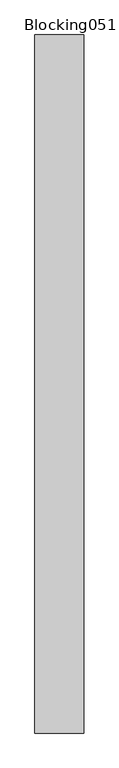
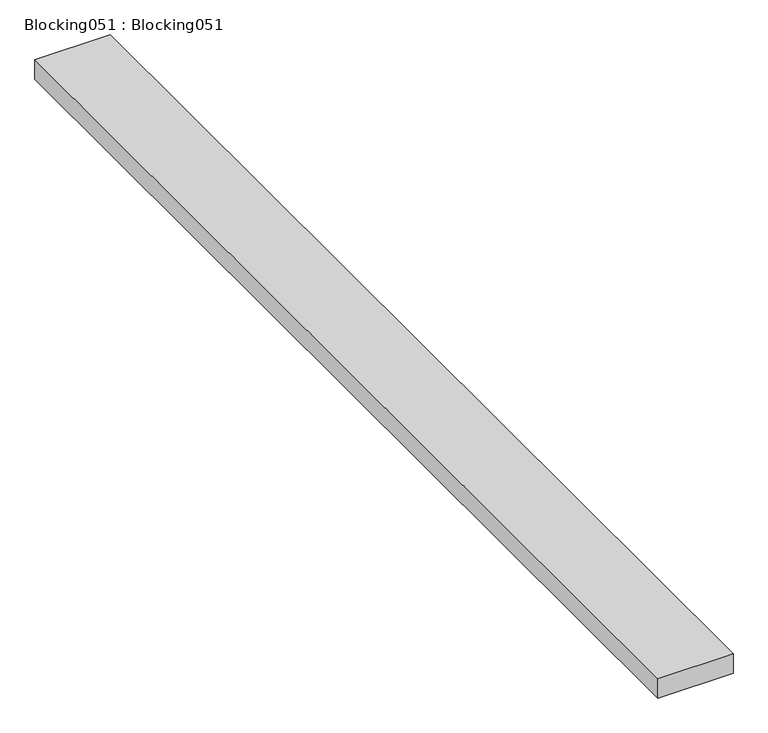
"""IFC4 building model written with IfcOpenShell, lengths in millimetres: proxy geometry, Blocking051 : Blocking051."""

import ifcopenshell
import ifcopenshell.guid

model = None  # the IFC model being written
_history = None  # IfcOwnerHistory: only IFC2X3 demands one
_inside = {}  # id of a spatial element -> (the spatial element, [elements in it])
_under = {}  # id of a project, library or spatial element -> (it, [spatial elements below it])
_declared = {}  # id of a project -> (the project, [libraries it declares])
_typed = {}  # id of a type object -> (the type object, [elements of that type])
_made_of = {}  # id of a material, layer set ... -> (it, [elements and type objects made of it])


def new_model(schema):
    """Start an empty IFC model of exactly this schema.

    Asked for "IFC4X3", IfcOpenShell would pick the latest addendum, in which some entities
    have other attributes; the version numbers below select the first issue.
    IFC2X3 requires an IfcOwnerHistory on every rooted entity: one is made here for all.
    """
    global model, _history
    if schema == "IFC4X3":
        model = ifcopenshell.file(schema_version=(4, 3, 0, 0))
    else:
        model = ifcopenshell.file(schema=schema)
    _inside.clear()
    _under.clear()
    _declared.clear()
    _typed.clear()
    _made_of.clear()
    _history = None
    if model.schema == "IFC2X3":
        org = make("IfcOrganization", Name="unknown")
        user = make(
            "IfcPersonAndOrganization",
            ThePerson=make("IfcPerson", FamilyName="unknown"),
            TheOrganization=org,
        )
        app = make(
            "IfcApplication",
            ApplicationDeveloper=org,
            Version="unknown",
            ApplicationFullName="unknown",
            ApplicationIdentifier="unknown",
        )
        _history = make(
            "IfcOwnerHistory",
            OwningUser=user,
            OwningApplication=app,
            ChangeAction="ADDED",
            CreationDate=0,
        )
    return model


def make(cls, **values):
    """One entity of the class cls with the attributes given. An attribute that is None is left unset."""
    return model.create_entity(
        cls, **{name: value for name, value in values.items() if value is not None}
    )


def rooted(cls, **values):
    """An entity with a GlobalId (a new one), such as an element, a storey or a relation."""
    return make(cls, GlobalId=ifcopenshell.guid.new(), OwnerHistory=_history, **values)


def si_unit(unit_type, name, prefix=None):
    """IfcSIUnit, for example si_unit("LENGTHUNIT", "METRE", prefix="MILLI")."""
    return make("IfcSIUnit", UnitType=unit_type, Prefix=prefix, Name=name)


def assignment(units):
    """IfcUnitAssignment: the units of a project."""
    return None if units is None else make("IfcUnitAssignment", Units=units)


def point(xyz):
    """IfcCartesianPoint."""
    return None if xyz is None else make("IfcCartesianPoint", Coordinates=xyz)


def direction(xyz):
    """IfcDirection."""
    return None if xyz is None else make("IfcDirection", DirectionRatios=xyz)


def frame(location, z_axis=None, x_axis=None):
    """IfcAxis2Placement3D, a coordinate frame: its origin and axes. An axis left out is left unset."""
    return make(
        "IfcAxis2Placement3D",
        Location=point(location),
        Axis=direction(z_axis),
        RefDirection=direction(x_axis),
    )


def origin():
    """The frame at (0, 0, 0) with its axes left unset."""
    return frame((0.0, 0.0, 0.0))


def place(relative_to, where):
    """IfcLocalPlacement: puts the frame where relative to a parent placement (None: the world)."""
    return make(
        "IfcLocalPlacement", PlacementRelTo=relative_to, RelativePlacement=where
    )


def context(
    kind, dimensions, precision=None, world=None, true_north=None, identifier=None
):
    """IfcGeometricRepresentationContext, for example the 3D "Model" context."""
    return make(
        "IfcGeometricRepresentationContext",
        ContextIdentifier=identifier,
        ContextType=kind,
        CoordinateSpaceDimension=dimensions,
        Precision=precision,
        WorldCoordinateSystem=world,
        TrueNorth=true_north,
    )


def project(units=None, contexts=None):
    """IfcProject with its units and contexts."""
    return rooted(
        "IfcProject",
        Name="project",
        RepresentationContexts=contexts,
        UnitsInContext=assignment(units),
    )


def spatial(cls, under=None, at=None, **own):
    """A site, building, storey or space (cls), placed at a placement, below another one or the project."""
    s = rooted(cls, ObjectPlacement=at, **own)
    if under is not None:
        _under.setdefault(under.id(), (under, []))[1].append(s)
    return s


def polyline(points):
    """IfcPolyline through the points."""
    return make("IfcPolyline", Points=[point(p) for p in points])


def outline(outer, holes=None, kind="AREA"):
    """IfcArbitraryClosedProfileDef: a profile drawn as a closed curve; with holes, ...WithVoids."""
    if holes is None:
        return make("IfcArbitraryClosedProfileDef", ProfileType=kind, OuterCurve=outer)
    return make(
        "IfcArbitraryProfileDefWithVoids",
        ProfileType=kind,
        OuterCurve=outer,
        InnerCurves=holes,
    )


def extrude(swept, where, along, depth):
    """IfcExtrudedAreaSolid: the profile swept, set in the frame where, extruded along a direction by depth."""
    return make(
        "IfcExtrudedAreaSolid",
        SweptArea=swept,
        Position=where,
        ExtrudedDirection=direction(along),
        Depth=depth,
    )


def shape(context_of_items, identifier, shape_type, items):
    """IfcShapeRepresentation: the items that make up one representation, for example the "Body"."""
    return make(
        "IfcShapeRepresentation",
        ContextOfItems=context_of_items,
        RepresentationIdentifier=identifier,
        RepresentationType=shape_type,
        Items=items,
    )


def source(mapping_origin, context_of_items, identifier, shape_type, items):
    """IfcRepresentationMap: a shape defined once, which mapped items show again and again."""
    return make(
        "IfcRepresentationMap",
        MappingOrigin=mapping_origin,
        MappedRepresentation=shape(context_of_items, identifier, shape_type, items),
    )


def transform(
    local_origin,
    x_axis=None,
    y_axis=None,
    z_axis=None,
    scale=None,
    scale2=None,
    scale3=None,
    uniform=True,
):
    """IfcCartesianTransformationOperator3D, or its non-uniform kind. x_axis, y_axis, z_axis: its Axis1, 2, 3."""
    if uniform:
        return make(
            "IfcCartesianTransformationOperator3D",
            Axis1=direction(x_axis),
            Axis2=direction(y_axis),
            LocalOrigin=point(local_origin),
            Scale=scale,
            Axis3=direction(z_axis),
        )
    return make(
        "IfcCartesianTransformationOperator3DnonUniform",
        Axis1=direction(x_axis),
        Axis2=direction(y_axis),
        LocalOrigin=point(local_origin),
        Scale=scale,
        Axis3=direction(z_axis),
        Scale2=scale2,
        Scale3=scale3,
    )


def mapped(mapping_source, mapping_target):
    """IfcMappedItem: shows the shape of a source again, moved by a transform."""
    return make(
        "IfcMappedItem", MappingSource=mapping_source, MappingTarget=mapping_target
    )


def made_of(thing, what):
    """Note that an element or type object is made of a material, layer set ...; save() writes the relation."""
    if what is not None:
        _made_of.setdefault(what.id(), (what, []))[1].append(thing)
    return thing


def element(
    cls,
    number,
    at=None,
    inside=None,
    cuts=None,
    type_object=None,
    material=None,
    context=None,
    identifier="Body",
    shape_type=None,
    held_by="IfcProductDefinitionShape",
    body=None,
    shapes=None,
    **own,
):
    """One element of the class cls, such as IfcWall. Its Tag is "e" and its number.

    at: its placement. inside: the storey or other place that contains it. cuts: it is an
    opening in that element (IfcRelVoidsElement). A single representation is given by context,
    identifier, shape_type and body (its items); several are given by shapes. held_by: the class
    of the entity that holds the representations. save() writes the other relations.
    """
    e = rooted(cls, Tag="e%d" % number, ObjectPlacement=at, **own)
    if body is not None:
        shapes = [shape(context, identifier, shape_type, body)]
    if shapes is not None:
        e.Representation = make(held_by, Representations=shapes)
    if inside is not None:
        _inside.setdefault(inside.id(), (inside, []))[1].append(e)
    if cuts is not None:
        rooted(
            "IfcRelVoidsElement", RelatingBuildingElement=cuts, RelatedOpeningElement=e
        )
    if type_object is not None:
        _typed.setdefault(type_object.id(), (type_object, []))[1].append(e)
    return made_of(e, material)


def aggregate(whole, parts):
    """IfcRelAggregates: a whole, such as a stair, and the parts it consists of."""
    return rooted("IfcRelAggregates", RelatingObject=whole, RelatedObjects=parts)


def save(model, path):
    """Write the relations noted so far, then the file.

    IfcRelAggregates (storeys below a building ...), IfcRelContainedInSpatialStructure (elements
    in a storey), IfcRelDefinesByType, IfcRelAssociatesMaterial and IfcRelDeclares: one each for
    every whole, place, type object, material and project.
    """
    for whole, parts in _under.values():
        aggregate(whole, parts)
    for where, things in _inside.values():
        rooted(
            "IfcRelContainedInSpatialStructure",
            RelatedElements=things,
            RelatingStructure=where,
        )
    for kind, things in _typed.values():
        rooted("IfcRelDefinesByType", RelatedObjects=things, RelatingType=kind)
    for what, things in _made_of.values():
        rooted("IfcRelAssociatesMaterial", RelatedObjects=things, RelatingMaterial=what)
    for by, libraries in _declared.values():
        rooted("IfcRelDeclares", RelatingContext=by, RelatedDefinitions=libraries)
    model.write(path)


def blocking051_blocking051_b2aed941(model_context):
    return source(origin(), model_context, "Body", "SweptSolid", [
        extrude(outline(polyline([(-9501.574441, 7982.1529359), (-9641.274441, 7982.1529359), (-9641.274441, 9982.1529359), (-9501.574441, 9982.1529359), (-9501.574441, 7982.1529359)])), frame((0.0, 0.0, 32606.9960253), z_axis=(0.0, 0.0, 1.0), x_axis=(1.0, 0.0, 0.0)), (0.0, 0.0, 1.0), 38.1),
    ])


if __name__ == "__main__":
    model = new_model("IFC4")
    model_context = context("Model", 3, world=origin())
    ifc_project = project(units=[si_unit("LENGTHUNIT", "METRE", prefix="MILLI")], contexts=[model_context])
    site = spatial("IfcSite", under=ifc_project)
    building = spatial("IfcBuilding", under=site)
    placement = place(None, origin())
    blocking051_blocking051_shape = blocking051_blocking051_b2aed941(model_context)
    element("IfcBuildingElementProxy", 1, Name="Blocking051 : Blocking051", ObjectType="Blocking051 : Blocking051", at=placement, inside=building, context=model_context, shape_type="MappedRepresentation", body=[
        mapped(blocking051_blocking051_shape, transform((0.0, 0.0, 0.0), x_axis=(1.0, 0.0, 0.0), y_axis=(0.0, 1.0, 0.0), z_axis=(0.0, 0.0, 1.0))),
    ])
    save(model, "model.ifc")

# Revit data of these elements
# Type "Blocking051 : Blocking051"
#   NameOverride = "Blocking051"
# Element 1 (IfcBuildingElementProxy, "Blocking051 : Blocking051")
#   Materials on its faces: "WOOD BLOCKING AS REQUIRED"
# Materials
#   "WOOD BLOCKING AS REQUIRED": class "Unassigned", colour RGB 166 124 85, transparency 0, Cost = 0
